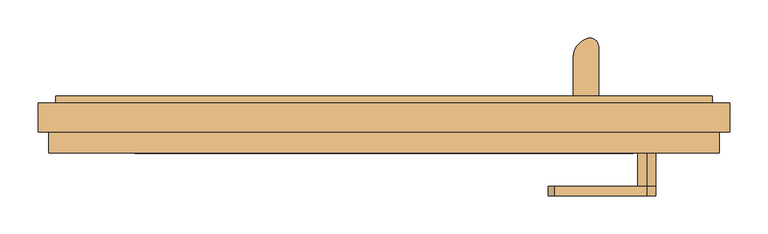
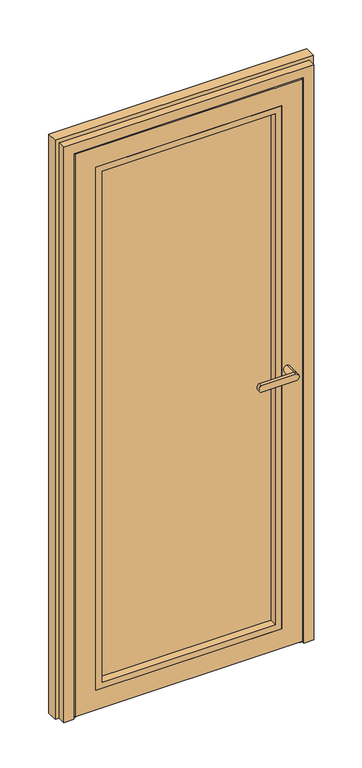
"""IFC4 building model written with IfcOpenShell, lengths in millimetres: door geometry, Schueco_FWS_ADS-75-HD-HI_inw_Family-01 : FWS SI insert unit."""

from ifc_helpers import new_model, si_unit, point, frame, frame_2d, origin, place, context, project, spatial, polyline, circle_curve, ellipse_curve, trimmed, segment, composite_curve, outline, extrude, faceted_brep, source, transform, mapped, element, save
from ifc_brep_helpers import plane_surface, cylinder_surface, extruded_surface, advanced_brep


def door_e4dfd9d4(model_context):
    return source(origin(), model_context, "Body", "SolidModel", [
        extrude(outline(composite_curve([segment(polyline([(248.3337564, 8.9997177), (248.3337564, 59.1618682)]), True, "CONTINUOUS"), segment(trimmed(circle_curve(frame_2d((275.512174, 59.1618682)), 27.1784177), [point((248.3337564, 59.1618682))], [point((265.9750784, 84.6120194))], False, "CARTESIAN"), True, "CONTINUOUS"), segment(trimmed(circle_curve(frame_2d((270.0525794, 73.7310321)), 11.6198924), [point((265.9750784, 84.6120194))], [point((281.6724718, 73.7310321))], False, "CARTESIAN"), True, "CONTINUOUS"), segment(polyline([(281.6724718, 73.7310321), (281.6724718, 8.9997177), (248.3337564, 8.9997177)]), True, "CONTINUOUS")], self_intersect=False)), frame((0.0, 0.0, 2053.9218203), z_axis=(0.0, 0.0, 1.0), x_axis=(1.0, 0.0, 0.0)), (0.0, 0.0, 1.0), 4.0),
        extrude(outline(polyline([(248.3337564, 12.9997177), (281.6724718, 12.9997177), (281.6724718, 8.9997177), (248.3337564, 8.9997177), (248.3337564, 12.9997177)])), frame((0.0, 0.0, 2023.9218203), z_axis=(0.0, 0.0, 1.0), x_axis=(1.0, 0.0, 0.0)), (0.0, 0.0, 1.0), 30.0),
        extrude(outline(polyline([(248.3337564, 12.9997177), (281.6724718, 12.9997177), (281.6724718, 8.9997177), (248.3337564, 8.9997177), (248.3337564, 12.9997177)])), frame((0.0, 0.0, 49.9218203), z_axis=(0.0, 0.0, 1.0), x_axis=(1.0, 0.0, 0.0)), (0.0, 0.0, 1.0), 30.0),
        extrude(outline(composite_curve([segment(polyline([(248.3337564, 8.9997177), (248.3337564, 59.1618682)]), True, "CONTINUOUS"), segment(trimmed(circle_curve(frame_2d((275.512174, 59.1618682)), 27.1784177), [point((248.3337564, 59.1618682))], [point((265.9750784, 84.6120194))], False, "CARTESIAN"), True, "CONTINUOUS"), segment(trimmed(circle_curve(frame_2d((270.0525794, 73.7310321)), 11.6198924), [point((265.9750784, 84.6120194))], [point((281.6724718, 73.7310321))], False, "CARTESIAN"), True, "CONTINUOUS"), segment(polyline([(281.6724718, 73.7310321), (281.6724718, 8.9997177), (248.3337564, 8.9997177)]), True, "CONTINUOUS")], self_intersect=False)), frame((0.0, 0.0, 45.9218203), z_axis=(0.0, 0.0, 1.0), x_axis=(1.0, 0.0, 0.0)), (0.0, 0.0, 1.0), 4.0),
        advanced_brep(
        [(277.718156, 57.5977179, 2053.9218203), (252.2840039, 72.2821425, 2053.9218203), (277.718156, 57.5977179, 49.9218203), (252.2840039, 72.2821425, 49.9218203)],
        [
            (0, 1, ellipse_curve(frame((265.0010799, 64.9399302, 2053.9218203), z_axis=(0.0, 0.0, 1.0000000000000002), x_axis=(0.5000002582658958, 0.866025254674503, 0.0)), 21.5840887, 14.6844171)),
            (1, 0, ellipse_curve(frame((265.0010799, 64.9399302, 2053.9218203), z_axis=(0.0, 0.0, 1.0000000000000002), x_axis=(0.5000002582658958, 0.866025254674503, 0.0)), 21.5840887, 14.6844171)),
            (2, 3, ellipse_curve(frame((265.0010799, 64.9399302, 49.9218203), z_axis=(0.0, 0.0, -1.0000000000000002), x_axis=(-0.866025254674503, 0.5000002582658958, 0.0)), 14.6844171, 21.5840887)),
            (3, 2, ellipse_curve(frame((265.0010799, 64.9399302, 49.9218203), z_axis=(0.0, 0.0, -1.0000000000000002), x_axis=(-0.866025254674503, 0.5000002582658958, 0.0)), 14.6844171, 21.5840887)),
            (0, 2),
            (3, 1),
        ],
        [
            plane_surface(frame((252.2840039, 72.2821425, 2053.9218203), z_axis=(0.0, 0.0, 1.0000000000000002), x_axis=(0.5000002582658958, 0.866025254674503, 0.0))),
            plane_surface(frame((252.2840039, 72.2821425, 49.9218203), z_axis=(0.0, 0.0, -1.0000000000000002), x_axis=(-0.5000002582658958, -0.866025254674503, 0.0))),
            extruded_surface(trimmed(ellipse_curve(frame((265.0010799, 64.9399302, 49.9218203), z_axis=(0.0, 0.0, -1.0000000000000002), x_axis=(-0.866025254674503, 0.5000002582658958, 0.0)), 14.6844171, 21.5840887), [point((252.2840039, 72.2821425, 49.9218203))], [point((277.718156, 57.5977179, 49.9218203))], True, "CARTESIAN"), (0.0, 0.0, -2004.0), 2004.0),
            extruded_surface(trimmed(ellipse_curve(frame((265.0010799, 64.9399302, 49.9218203), z_axis=(0.0, 0.0, -1.0000000000000002), x_axis=(-0.866025254674503, 0.5000002582658958, 0.0)), 14.6844171, 21.5840887), [point((277.718156, 57.5977179, 49.9218203))], [point((252.2840039, 72.2821425, 49.9218203))], True, "CARTESIAN"), (0.0, 0.0, -2004.0), 2004.0),
        ],
        [
            (0, [[1, 2]]),
            (1, [[3, 4]]),
            (2, [[5, -4, 6, -1]]),
            (3, [[-6, -3, -5, -2]]),
        ],
    ),
        advanced_brep(
        [(345.0010799, -122.0002518, 1030.9991882), (345.0010799, -122.0002518, 1054.9764498), (223.3392873, -122.0002518, 1054.9764498), (223.3392873, -122.0002518, 1030.9991882), (345.0010799, -109.5001648, 1054.9764498), (345.0010799, -109.5001648, 1030.9991882), (223.3392873, -109.5001648, 1030.9991882), (223.3392873, -109.5001648, 1054.9764498), (345.0010799, -66.0002823, 1030.9991882), (345.0010799, -66.0002823, 1054.9764498)],
        [
            (0, 1, circle_curve(frame((345.0010799, -122.0002518, 1042.987819), z_axis=(0.0, -1.0, 0.0), x_axis=(0.0, 0.0, 1.0)), 11.9886308)),
            (1, 2),
            (2, 3, ellipse_curve(frame((223.3392873, -122.0002518, 1042.987819), z_axis=(0.0, -1.0, 0.0), x_axis=(0.0, 0.0, -1.0)), 11.9886308, 7.9050795)),
            (3, 0),
            (4, 5, circle_curve(frame((345.0010799, -109.5001648, 1042.987819), z_axis=(0.0, -1.0, 0.0), x_axis=(0.0, 0.0, 1.0)), 11.9886308)),
            (5, 6),
            (6, 7, ellipse_curve(frame((223.3392873, -109.5001648, 1042.987819), z_axis=(0.0, 1.0, 0.0), x_axis=(0.0, 0.0, -1.0)), 11.9886308, 7.9050795)),
            (7, 4),
            (3, 6),
            (5, 0),
            (2, 7),
            (1, 4),
            (5, 4, circle_curve(frame((345.0010799, -109.5001648, 1042.987819), z_axis=(0.0, -1.0, 0.0), x_axis=(0.0, 0.0, 1.0)), 11.9886308)),
            (8, 9, circle_curve(frame((345.0010799, -66.0002823, 1042.987819), z_axis=(0.0, 1.0, 0.0), x_axis=(0.0, 0.0, 1.0)), 11.9886308)),
            (9, 8, circle_curve(frame((345.0010799, -66.0002823, 1042.987819), z_axis=(0.0, 1.0, 0.0), x_axis=(0.0, 0.0, 1.0)), 11.9886308)),
            (8, 5),
            (4, 9),
        ],
        [
            plane_surface(frame((223.3392873, -122.0002518, 1030.9991882), z_axis=(0.0, -1.0, 0.0), x_axis=(-1.0, 0.0, 0.0))),
            plane_surface(frame((223.3392873, -109.5001648, 1030.9991882), z_axis=(0.0, 1.0, 0.0), x_axis=(1.0, 0.0, 0.0))),
            plane_surface(frame((345.0010799, -122.0002518, 1030.9991882), z_axis=(0.0, 0.0, -1.0), x_axis=(0.0, 1.0, 0.0))),
            extruded_surface(trimmed(ellipse_curve(frame((223.3392873, -109.5001648, 1042.987819), z_axis=(0.0, 1.0, 0.0), x_axis=(0.0, 0.0, -1.0)), 11.9886308, 7.9050795), [point((223.3392873, -109.5001648, 1030.9991882))], [point((223.3392873, -109.5001648, 1054.9764498))], True, "CARTESIAN"), (0.0, 12.500086999999994, 0.0), 12.500086999999994),
            plane_surface(frame((223.3392873, -122.0002518, 1054.9764498), z_axis=(0.0, 0.0, 1.0), x_axis=(0.0, 1.0, 0.0))),
            cylinder_surface(frame((345.0010799, -109.5001648, 1042.987819), z_axis=(0.0, -1.0, 0.0), x_axis=(0.0, 0.0, 1.0)), 11.9886308),
            plane_surface(frame((345.0010799, -66.0002823, 1054.9764498), z_axis=(0.0, 1.0, 0.0), x_axis=(-1.0, 0.0, 0.0))),
            cylinder_surface(frame((345.0010799, -66.0002823, 1042.987819), z_axis=(0.0, -1.0, 0.0), x_axis=(0.0, 0.0, 1.0)), 11.9886308),
        ],
        [
            (0, [[1, 2, 3, 4]]),
            (1, [[5, 6, 7, 8]]),
            (2, [[9, -6, 10, -4]]),
            (3, [[11, -7, -9, -3]]),
            (4, [[12, -8, -11, -2]]),
            (5, [[-10, 13, -12, -1]]),
            (6, [[14, 15]]),
            (7, [[16, -5, 17, -14]]),
            (7, [[-17, -13, -16, -15]]),
        ],
    ),
        extrude(outline(polyline([(80.9218203, 327.0670787), (2027.0538178, 327.0670787), (2027.0538178, -327.0649188), (80.9218203, -327.0649188), (80.9218203, 327.0670787)]), holes=[polyline([(102.9234681, -305.063271), (2005.05217, -305.063271), (2005.05217, 305.0654309), (102.9234681, 305.0654309), (102.9234681, -305.063271)])]), frame((0.0, -66.0002823, 0.0), z_axis=(0.0, 1.0, 0.0), x_axis=(0.0, 0.0, 1.0)), (0.0, 0.0, 1.0), 28.0002823),
        faceted_brep([(-399.9989201, -66.0002823, 2099.987819), (-399.9989201, -57.5000065, 2099.987819), (-399.9989201, -57.5000065, 7.987819), (-399.9989201, -66.0002823, 7.987819), (400.0010799, -57.5000065, 7.987819), (400.0010799, -66.0002823, 7.987819), (400.0010799, -57.5000065, 2099.987819), (385.0670787, -57.5000065, 22.9218203), (385.0670787, -57.5000065, 2085.0538178), (-385.0649188, -57.5000065, 2085.0538178), (-385.0649188, -57.5000065, 22.9218203), (400.0010799, -66.0002823, 2099.987819), (-327.0649188, -66.0002823, 80.9218203), (-327.0649188, -66.0002823, 2027.0538178), (327.0670787, -66.0002823, 2027.0538178), (327.0670787, -66.0002823, 80.9218203), (-327.0649188, 0.0, 2027.0538178), (-327.0649188, 0.0, 80.9218203), (327.0670787, 0.0, 80.9218203), (327.0670787, 0.0, 2027.0538178), (-302.0649188, 0.0, 105.9218203), (-302.0649188, 0.0, 2002.0538178), (302.0670787, 0.0, 2002.0538178), (302.0670787, 0.0, 105.9218203), (-302.0649188, 8.9997177, 2002.0538178), (-302.0649188, 8.9997177, 105.9218203), (302.0670787, 8.9997177, 105.9218203), (302.0670787, 8.9997177, 2002.0538178), (-375.0649188, 8.9997177, 32.9218203), (-375.0649188, 8.9997177, 2075.0538178), (375.0670787, 8.9997177, 2075.0538178), (375.0670787, 8.9997177, 32.9218203), (-375.0649188, 0.4997603, 2075.0538178), (-375.0649188, 0.4997603, 32.9218203), (375.0670787, 0.4997603, 32.9218203), (375.0670787, 0.4997603, 2075.0538178), (-385.0649188, 0.4997603, 22.9218203), (-385.0649188, 0.4997603, 2085.0538178), (385.0670787, 0.4997603, 2085.0538178), (385.0670787, 0.4997603, 22.9218203)], [[[0, 1, 2, 3]], [[3, 2, 4, 5]], [[2, 1, 6, 4], [7, 8, 9, 10]], [[5, 4, 6, 11]], [[5, 11, 0, 3], [12, 13, 14, 15]], [[16, 13, 12, 17]], [[17, 12, 15, 18]], [[18, 15, 14, 19]], [[18, 19, 16, 17], [20, 21, 22, 23]], [[24, 21, 20, 25]], [[25, 20, 23, 26]], [[26, 23, 22, 27]], [[28, 29, 30, 31], [26, 27, 24, 25]], [[32, 29, 28, 33]], [[33, 28, 31, 34]], [[34, 31, 30, 35]], [[36, 37, 38, 39], [34, 35, 32, 33]], [[9, 37, 36, 10]], [[10, 36, 39, 7]], [[7, 39, 38, 8]], [[11, 6, 1, 0]], [[19, 14, 13, 16]], [[27, 22, 21, 24]], [[35, 30, 29, 32]], [[8, 38, 37, 9]]]),
        extrude(outline(polyline([(327.0670787, -38.0), (-327.0649188, -38.0), (-327.0649188, 0.0), (327.0670787, 0.0), (327.0670787, -38.0)])), frame((0.0, 0.0, 80.9218203), z_axis=(0.0, 0.0, 1.0), x_axis=(1.0, 0.0, 0.0)), (0.0, 0.0, 1.0), 1946.1319975),
        extrude(outline(polyline([(-375.0649188, 0.4997603), (-375.0649188, 8.9997177), (375.0670787, 8.9997177), (375.0670787, 0.4997603), (-375.0649188, 0.4997603)])), frame((0.0, 0.0, 7.9218203), z_axis=(0.0, 0.0, 1.0), x_axis=(1.0, 0.0, 0.0)), (0.0, 0.0, 1.0), 25.0),
        extrude(outline(polyline([(-385.0649188, -28.5002397), (-385.0649188, -2.5002397), (385.0670787, -2.5002397), (385.0670787, -28.5002397), (-385.0649188, -28.5002397)])), frame((0.0, 0.0, 7.9218203), z_axis=(0.0, 0.0, 1.0), x_axis=(1.0, 0.0, 0.0)), (0.0, 0.0, 1.0), 15.0),
        faceted_brep([(430.999943, 8.9997177, 2130.999943), (430.999943, 0.0, 2130.999943), (430.999943, 0.0, 0.0), (430.999943, 8.9997177, 0.0), (-454.0, 0.0, 0.0), (-454.0, 0.0, 2154.0), (454.0, 0.0, 2154.0), (454.0, 0.0, 0.0), (-430.999943, 0.0, 2130.999943), (-430.999943, 0.0, 0.0), (454.0, -38.0, 0.0), (440.0, -38.0, 0.0), (440.0, -66.0002823, 0.0), (404.9999411, -66.0002823, 0.0), (404.9999411, -57.5000065, 0.0), (394.9999487, -57.5000065, 0.0), (394.9999487, 0.4997603, 0.0), (379.9999888, 0.4997603, 0.0), (379.9999888, 8.9997177, 0.0), (-379.9999888, 8.9997177, 0.0), (-430.999943, 8.9997177, 0.0), (-430.999943, 8.9997177, 2130.999943), (379.9999888, 8.9997177, 2079.9999888), (-379.9999888, 8.9997177, 2079.9999888), (404.9999411, -66.0002823, 2104.9999411), (404.9999411, -57.5000065, 2104.9999411), (-404.9999411, -57.5000065, 0.0), (-394.9999487, -57.5000065, 0.0), (-394.9999487, -57.5000065, 2094.9999487), (394.9999487, -57.5000065, 2094.9999487), (-404.9999411, -57.5000065, 2104.9999411), (-440.0, -66.0002823, 0.0), (-404.9999411, -66.0002823, 0.0), (-404.9999411, -66.0002823, 2104.9999411), (440.0, -66.0002823, 2140.0), (-440.0, -66.0002823, 2140.0), (440.0, -38.0, 2140.0), (-454.0, -38.0, 0.0), (-440.0, -38.0, 0.0), (-440.0, -38.0, 2140.0), (454.0, -38.0, 2154.0), (-454.0, -38.0, 2154.0), (-379.9999888, 0.4997603, 0.0), (-394.9999487, 0.4997603, 0.0), (379.9999888, 0.4997603, 2079.9999888), (-379.9999888, 0.4997603, 2079.9999888), (394.9999487, 0.4997603, 2094.9999487), (-394.9999487, 0.4997603, 2094.9999487)], [[[0, 1, 2, 3]], [[4, 5, 6, 7, 2, 1, 8, 9]], [[3, 2, 7, 10, 11, 12, 13, 14, 15, 16, 17, 18]], [[19, 20, 21, 0, 3, 18, 22, 23]], [[24, 25, 14, 13]], [[26, 27, 28, 29, 15, 14, 25, 30]], [[31, 32, 33, 24, 13, 12, 34, 35]], [[34, 12, 11, 36]], [[37, 38, 39, 36, 11, 10, 40, 41]], [[4, 9, 20, 19, 42, 43, 27, 26, 32, 31, 38, 37]], [[20, 9, 8, 21]], [[18, 17, 44, 22]], [[42, 19, 23, 45]], [[32, 26, 30, 33]], [[31, 35, 39, 38]], [[4, 37, 41, 5]], [[6, 40, 10, 7]], [[43, 42, 45, 44, 17, 16, 46, 47]], [[16, 15, 29, 46]], [[27, 43, 47, 28]], [[21, 8, 1, 0]], [[33, 30, 25, 24]], [[35, 34, 36, 39]], [[23, 22, 44, 45]], [[5, 41, 40, 6]], [[47, 46, 29, 28]]]),
        extrude(outline(polyline([(-1.3004128, 2.5), (-1.3004128, 0.0), (-55.3004128, 0.0), (-55.3004128, 2.5), (-43.0185552, 4.5), (-13.5822704, 4.5), (-1.3004128, 2.5)])), frame((-394.9999487, 0.0, 0.0), z_axis=(1.0, 0.0, 0.0), x_axis=(0.0, 1.0, 0.0)), (0.0, 0.0, 1.0), 789.9998975),
    ])


if __name__ == "__main__":
    model = new_model("IFC4")
    model_context = context("Model", 3, world=origin())
    ifc_project = project(units=[si_unit("LENGTHUNIT", "METRE", prefix="MILLI")], contexts=[model_context])
    site = spatial("IfcSite", under=ifc_project)
    building = spatial("IfcBuilding", under=site)
    placement = place(None, origin())
    door_shape = door_e4dfd9d4(model_context)
    element("IfcDoor", 1, ObjectType="Schueco_FWS_ADS-75-HD-HI_inw_Family-01 : FWS SI insert unit", at=placement, inside=building, context=model_context, shape_type="MappedRepresentation", body=[
        mapped(door_shape, transform((0.0, 0.0, 0.0), x_axis=(1.0, 0.0, 0.0), y_axis=(0.0, 1.0, 0.0), z_axis=(0.0, 0.0, 1.0))),
    ])
    save(model, "model.ifc")

# Revit data of these elements
# Type "Schueco_FWS_ADS-75-HD-HI_inw_Family-01 : FWS SI insert unit"
#   Type Mark = "25"
#   __NOTE__ = "Data describes the optimum values of the entire system. The properites of a selected design option have to be determined on an individual basis!"
#   Wind load resistance = "Class 2"
#   Watertightness = "Class 5A"
#   Thermal insulation = "Uf = 1.4 W/(m²K)"
#   Sound insulation = "to RW 43 db"
#   Schueco thermal insulation standard = "Highly thermally insulated"
#   Opening type = "Inward-opening, Flush-fitted"
#   Model = "Schueco ADS 75 HD.HI"
#   Mechanical loading = "Class 2"
#   Maximum leaf width in mm = "1400"
#   Maximum leaf weight in kg = "200"
#   Maximum leaf height in mm = "3000"
#   Material = "Aluminium"
#   Construction Type = "Door, single-leaf, inward-opening"
#   Manufacturer = "Schueco International KG"
#   Long term functionality = "Class 6"
#   Glazing data = "Triple glazing 38mm"
#   Façade insert unit = "yes"
#   Family creation date = "08.2017"
#   Description = "Schueco Aluminium Door System (ADS)"
#   Burglar resistance = "Class RC 3"
#   Areas of use = "Public buildings"
#   Analytic Construction = "<None>"
#   Air permeability = "Class 2"
#   Width [instance default] = 577.43 mm
#   Leaf opening angle [instance default] = 0.00°
#   IOf_T = 38 mm
#   Height [instance default] = 2219.367 mm
#   Glazing area [instance default] = 0.536296 m²
#   Distance from bottom to handles [instance default] = 1050 mm
#   Clear opening width [instance default] = 429.43 mm
#   Standard threshold = no
#   Low level threshold = yes
#   Handles = yes
#   FWS SI insert unit = yes
#   FWS HI insert unit = no
#   Glass = none
#   Frame = Alu
#   Fittings = none
# Element 1 (IfcDoor, "Schueco_FWS_ADS-75-HD-HI_inw_Family-01 : FWS SI insert unit")
#   Width = 908 mm
#   Height = 2154 mm
#   Glazing area = 1.14518 m²
#   Clear opening width = 760 mm
#   Materials on its faces: "Alu", "Glass"
# Materials
#   "Alu": class "Glas", colour RGB 140 140 140, transparency 0
#   "Glass": class "Glass", colour RGB 128 128 255, transparency 0.75, Description = "Soda Lime Glass", Cost = 0
